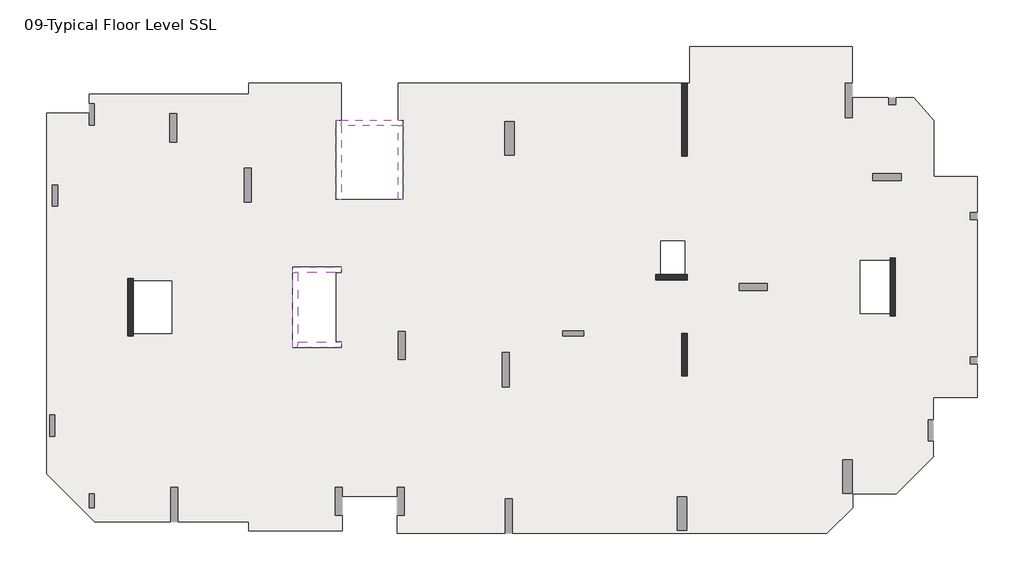
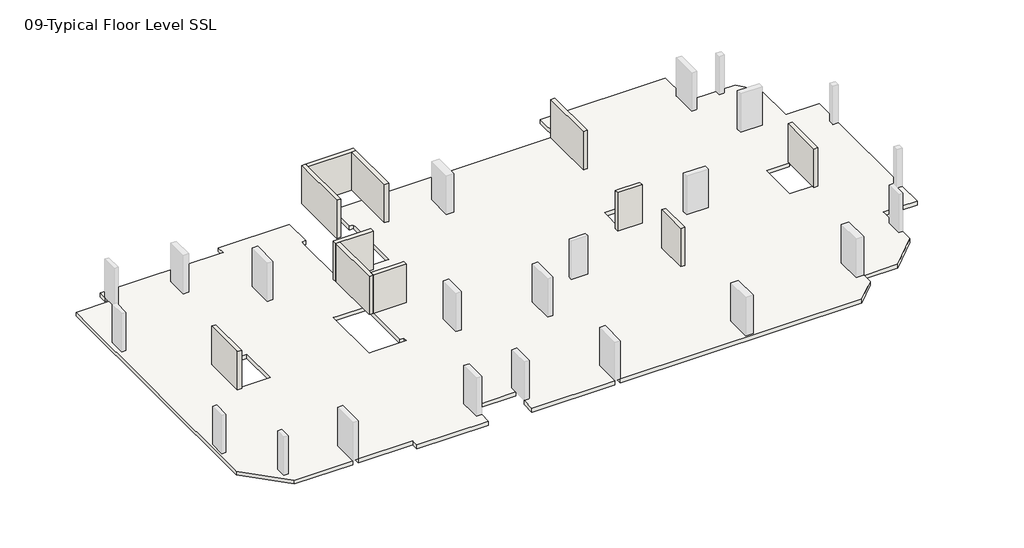
# One storey, part 1 of 2: 11 walls, 1 slab.
"""IFC4 building model written with IfcOpenShell, lengths in millimetres."""

from ifc_helpers import new_model, si_unit, origin, place, context, project, spatial, faceted_brep, element, save

model = new_model("IFC4")

# Units and contexts
model_context = context("Model", 3, world=origin())
ifc_project = project(units=[si_unit("LENGTHUNIT", "METRE", prefix="MILLI")], contexts=[model_context])

# Site, building, storey
site = spatial("IfcSite", under=ifc_project)
building = spatial("IfcBuilding", under=site)
storey = spatial("IfcBuildingStorey", under=building, Name="09-Typical Floor Level SSL", Elevation=21000.0)

# Slab
placement = place(None, origin())
element("IfcSlab", 1, ObjectType="Generic 300mm", at=placement, inside=storey, context=model_context, shape_type="Brep", body=[
    faceted_brep([(36192.0021644, 24072.000519, 20700.0), (36192.0021644, 26172.000519, 20700.0), (45446.0007483, 26172.000519, 20700.0), (45446.0007483, 24087.0, 20700.0), (45046.0007483, 24087.0, 20700.0), (45046.0007483, 22137.0, 20700.0), (45446.0007483, 22137.0, 20700.0), (45446.0007483, 23252.0000315, 20700.0), (47498.6337868, 23252.0000315, 20700.0), (47498.6337868, 22852.0, 20700.0), (47898.6337868, 22852.0, 20700.0), (47898.6337868, 23252.0000315, 20700.0), (48936.764334, 23252.0000315, 20700.0), (50076.0016214, 21956.8283806, 20700.0), (50076.0016214, 18780.0084406, 20700.0), (52549.9999998, 18780.0084406, 20700.0), (52549.9999998, 16712.0, 20700.0), (52149.9999998, 16712.0, 20700.0), (52149.9999998, 16312.0, 20700.0), (52549.9999998, 16312.0, 20700.0), (52549.9999998, 8504.0039609, 20700.0), (52149.9999998, 8504.0039609, 20700.0), (52149.9999998, 8104.0039609, 20700.0), (52549.9999998, 8104.0039609, 20700.0), (52549.9999998, 6204.0084406, 20700.0), (50046.0009271, 6204.0084406, 20700.0), (50046.0009271, 4931.9999929, 20700.0), (49746.0009271, 4931.9999929, 20700.0), (49746.0009271, 3731.9999929, 20700.0), (50046.0009271, 3731.9999929, 20700.0), (50046.0009271, 2810.5958657, 20700.0), (47943.4055804, 708.000519, 20700.0), (45456.0017287, 708.000519, 20700.0), (45456.0017287, -61.7051085, 20700.0), (43990.7023722, -1527.004465, 20700.0), (26113.9999998, -1527.004465, 20700.0), (26113.9999998, 422.995535, 20700.0), (25713.9999998, 422.995535, 20700.0), (25713.9999998, -1527.004465, 20700.0), (19569.9997488, -1527.004465, 20700.0), (19569.9997488, -512.0044652, 20700.0), (19969.9997488, -512.0044652, 20700.0), (19969.9997488, 1087.9955348, 20700.0), (19569.9997488, 1087.9955348, 20700.0), (19569.9997488, 564.000519, 20700.0), (16429.9999981, 564.000519, 20700.0), (16429.9999981, 1088.0, 20700.0), (16029.9999981, 1088.0, 20700.0), (16029.9999981, -512.0, 20700.0), (16429.9999981, -512.0, 20700.0), (16429.9999981, -1391.999481, 20700.0), (11136.0000923, -1391.999481, 20700.0), (11136.0000923, -866.9999847, 20700.0), (7082.0000416, -866.9999847, 20700.0), (7082.0000416, 1083.0000153, 20700.0), (6682.0000416, 1083.0000153, 20700.0), (6682.0000416, -866.9999847, 20700.0), (2364.4419097, -866.9999847, 20700.0), (-372.0, 1869.441925, 20700.0), (-372.0, 22380.0004589, 20700.0), (2052.0, 22380.0004589, 20700.0), (2052.0, 21708.0000656, 20700.0), (2352.0, 21708.0000656, 20700.0), (2352.0, 22908.0000656, 20700.0), (2052.0, 22908.0000656, 20700.0), (2052.0, 23472.000519, 20700.0), (11136.0000923, 23472.000519, 20700.0), (11136.0000923, 24072.000519, 20700.0), (16380.0000168, 24072.000519, 20700.0), (16380.0000168, 21972.0, 20700.0), (16079.9999997, 21972.0, 20700.0), (16079.9999997, 21672.0, 20700.0), (16079.9999997, 17468.0, 20700.0), (16379.9999997, 17468.0, 20700.0), (19619.9999997, 17468.0, 20700.0), (19919.9999997, 17468.0, 20700.0), (19919.9999997, 21672.0, 20700.0), (19919.9999997, 21972.0, 20700.0), (19619.9997365, 21972.0, 20700.0), (19619.9997365, 24072.000519, 20700.0), (35747.9999998, 24072.000519, 20700.0), (35747.9999998, 19932.0, 20700.0), (36047.9999998, 19932.0, 20700.0), (36047.9999998, 24072.000519, 20700.0), (16079.9999907, 9359.999998, 20700.0), (16079.9999907, 13320.0000002, 20700.0), (16380.0000168, 13320.0000002, 20700.0), (16380.0000168, 13620.0000002, 20700.0), (13919.9999907, 13620.0000002, 20700.0), (13619.9999907, 13620.0000002, 20700.0), (13619.9999907, 13320.0000002, 20700.0), (13619.9999907, 9359.999998, 20700.0), (13619.9999907, 9059.999998, 20700.0), (13919.9999907, 9059.999998, 20700.0), (16380.0000168, 9059.999998, 20700.0), (16380.0000168, 9359.999998, 20700.0), (4548.0000034, 9840.0000003, 20700.0), (6743.9999995, 9840.0000003, 20700.0), (6743.9999995, 12840.0000003, 20700.0), (4548.0000034, 12840.0000003, 20700.0), (4548.0000025, 12984.0000001, 20700.0), (4248.0000025, 12984.0000001, 20700.0), (4248.0000025, 9696.0, 20700.0), (4548.0000025, 9696.0, 20700.0), (47580.0014798, 13992.0079177, 20700.0), (45900.001729, 13992.0079177, 20700.0), (45900.001729, 10992.0079181, 20700.0), (47580.0014798, 10992.0079181, 20700.0), (47580.0014811, 10848.0079202, 20700.0), (47880.0014811, 10848.0079202, 20700.0), (47880.0014811, 14136.0000002, 20700.0), (47580.0014811, 14136.0000002, 20700.0), (35904.002157, 15108.0000083, 20700.0), (34548.0015145, 15108.0000083, 20700.0), (34548.0015145, 13199.9999992, 20700.0), (34248.0015201, 13199.9999992, 20700.0), (34248.0015201, 12899.9999992, 20700.0), (36048.0015201, 12899.9999992, 20700.0), (36048.0015201, 13199.9999992, 20700.0), (35904.002157, 13199.9999992, 20700.0), (257.9999999, 17088.0, 20700.0), (257.9999999, 18288.0, 20700.0), (-42.0000001, 18288.0, 20700.0), (-42.0000001, 17088.0, 20700.0), (108.001803, 4001.9999858, 20700.0), (108.001803, 5201.9999858, 20700.0), (-191.998197, 5201.9999858, 20700.0), (-191.998197, 4001.9999858, 20700.0), (30175.9999998, 9996.0000019, 20700.0), (28975.9999998, 9996.0000019, 20700.0), (28975.9999998, 9696.0000019, 20700.0), (30175.9999998, 9696.0000019, 20700.0), (7021.9999999, 20740.0000078, 20700.0), (7021.9999999, 22340.0000078, 20700.0), (6621.9999999, 22340.0000078, 20700.0), (6621.9999999, 20740.0000078, 20700.0), (48205.9993605, 18950.0, 20700.0), (46605.9993605, 18950.0, 20700.0), (46605.9993605, 18550.0, 20700.0), (48205.9993605, 18550.0, 20700.0), (20030.000009, 8355.9999979, 20700.0), (20030.000009, 9955.9999979, 20700.0), (19630.000009, 9955.9999979, 20700.0), (19630.000009, 8355.9999979, 20700.0), (11270.0000427, 17312.9999996, 20700.0), (11270.0000427, 19262.9999996, 20700.0), (10870.0000427, 19262.9999996, 20700.0), (10870.0000427, 17312.9999996, 20700.0), (40598.0014887, 12692.0079212, 20700.0), (38998.0014887, 12692.0079212, 20700.0), (38998.0014887, 12292.0079212, 20700.0), (40598.0014887, 12292.0079212, 20700.0), (2352.0, -72.0, 20700.0), (2352.0, 728.0, 20700.0), (2052.0, 728.0, 20700.0), (2052.0, -72.0, 20700.0), (25934.0000455, 6801.0001824, 20700.0), (25934.0000455, 8751.0001824, 20700.0), (25534.0000455, 8751.0001824, 20700.0), (25534.0000455, 6801.0001824, 20700.0), (36035.9999998, -1351.9992017, 20700.0), (36035.9999998, 548.0007983, 20700.0), (35485.9999998, 548.0007983, 20700.0), (35485.9999998, -1351.9992017, 20700.0), (45443.9999998, 748.0, 20700.0), (45443.9999998, 2648.0, 20700.0), (44893.9999998, 2648.0, 20700.0), (44893.9999998, 748.0, 20700.0), (26218.9999998, 20000.0, 20700.0), (26218.9999998, 21900.0, 20700.0), (25668.9999998, 21900.0, 20700.0), (25668.9999998, 20000.0, 20700.0), (35748.0054035, 9840.0000002, 20700.0), (35748.0054035, 7428.0000762, 20700.0), (36048.0054035, 7428.0000762, 20700.0), (36048.0054035, 9840.0000002, 20700.0), (36192.0021644, 26172.000519, 21000.0), (36192.0021644, 24072.000519, 21000.0), (36047.9999998, 24072.000519, 21000.0), (36047.9999998, 19932.0, 21000.0), (35747.9999998, 19932.0, 21000.0), (35747.9999998, 24072.000519, 21000.0), (19619.9997365, 24072.000519, 21000.0), (19619.9997365, 21972.0, 21000.0), (19919.9999997, 21972.0, 21000.0), (19919.9999997, 21672.0, 21000.0), (19919.9999997, 17468.0, 21000.0), (19619.9999997, 17468.0, 21000.0), (16379.9999997, 17468.0, 21000.0), (16079.9999997, 17468.0, 21000.0), (16079.9999997, 21672.0, 21000.0), (16079.9999997, 21972.0, 21000.0), (16380.0000168, 21972.0, 21000.0), (16380.0000168, 24072.000519, 21000.0), (11136.0000923, 24072.000519, 21000.0), (11136.0000923, 23472.000519, 21000.0), (2052.0, 23472.000519, 21000.0), (2052.0, 22908.0000656, 21000.0), (2352.0, 22908.0000656, 21000.0), (2352.0, 21708.0000656, 21000.0), (2052.0, 21708.0000656, 21000.0), (2052.0, 22380.0004589, 21000.0), (-372.0, 22380.0004589, 21000.0), (-372.0, 1869.441925, 21000.0), (2364.4419097, -866.9999847, 21000.0), (6682.0000416, -866.9999847, 21000.0), (6682.0000416, 1083.0000153, 21000.0), (7082.0000416, 1083.0000153, 21000.0), (7082.0000416, -866.9999847, 21000.0), (11136.0000923, -866.9999847, 21000.0), (11136.0000923, -1391.999481, 21000.0), (16429.9999981, -1391.999481, 21000.0), (16429.9999981, -512.0, 21000.0), (16029.9999981, -512.0, 21000.0), (16029.9999981, 1088.0, 21000.0), (16429.9999981, 1088.0, 21000.0), (16429.9999981, 564.000519, 21000.0), (19569.9997488, 564.000519, 21000.0), (19569.9997488, 1087.9955348, 21000.0), (19969.9997488, 1087.9955348, 21000.0), (19969.9997488, -512.0044652, 21000.0), (19569.9997488, -512.0044652, 21000.0), (19569.9997488, -1527.004465, 21000.0), (25713.9999998, -1527.004465, 21000.0), (25713.9999998, 422.995535, 21000.0), (26113.9999998, 422.995535, 21000.0), (26113.9999998, -1527.004465, 21000.0), (43990.7023722, -1527.004465, 21000.0), (45456.0017287, -61.7051085, 21000.0), (45456.0017287, 708.000519, 21000.0), (47943.4055804, 708.000519, 21000.0), (50046.0009271, 2810.5958657, 21000.0), (50046.0009271, 3731.9999929, 21000.0), (49746.0009271, 3731.9999929, 21000.0), (49746.0009271, 4931.9999929, 21000.0), (50046.0009271, 4931.9999929, 21000.0), (50046.0009271, 6204.0084406, 21000.0), (52549.9999998, 6204.0084406, 21000.0), (52549.9999998, 8104.0039609, 21000.0), (52149.9999998, 8104.0039609, 21000.0), (52149.9999998, 8504.0039609, 21000.0), (52549.9999998, 8504.0039609, 21000.0), (52549.9999998, 16312.0, 21000.0), (52149.9999998, 16312.0, 21000.0), (52149.9999998, 16712.0, 21000.0), (52549.9999998, 16712.0, 21000.0), (52549.9999998, 18780.0084406, 21000.0), (50076.0016214, 18780.0084406, 21000.0), (50076.0016214, 21956.8283806, 21000.0), (48936.764334, 23252.0000315, 21000.0), (47898.6337868, 23252.0000315, 21000.0), (47898.6337868, 22852.0, 21000.0), (47498.6337868, 22852.0, 21000.0), (47498.6337868, 23252.0000315, 21000.0), (45446.0006898, 23252.0000315, 21000.0), (45446.0007483, 22137.0, 21000.0), (45046.0007483, 22137.0, 21000.0), (45046.0007483, 24087.0, 21000.0), (45446.0007483, 24087.0, 21000.0), (45446.0007483, 26172.000519, 21000.0), (16079.9999907, 13320.0000002, 21000.0), (16079.9999907, 9359.999998, 21000.0), (16380.0000168, 9359.999998, 21000.0), (16380.0000168, 9059.999998, 21000.0), (13919.9999907, 9059.999998, 21000.0), (13619.9999907, 9059.999998, 21000.0), (13619.9999907, 9359.999998, 21000.0), (13619.9999907, 13320.0000002, 21000.0), (13619.9999907, 13620.0000002, 21000.0), (13919.9999907, 13620.0000002, 21000.0), (16380.0000168, 13620.0000002, 21000.0), (16380.0000168, 13320.0000002, 21000.0), (6743.9999995, 9840.0000003, 21000.0), (4548.0000034, 9840.0000003, 21000.0), (4548.0000025, 9696.0, 21000.0), (4248.0000025, 9696.0, 21000.0), (4248.0000025, 12984.0000001, 21000.0), (4548.0000025, 12984.0000001, 21000.0), (4548.0000025, 12840.0000003, 21000.0), (6743.9999995, 12840.0000003, 21000.0), (45900.001729, 13992.0079177, 21000.0), (47580.0014798, 13992.0079177, 21000.0), (47580.0014811, 14136.0000002, 21000.0), (47880.0014811, 14136.0000002, 21000.0), (47880.0014811, 10848.0079202, 21000.0), (47580.0014811, 10848.0079202, 21000.0), (47580.0014811, 10992.0079181, 21000.0), (45900.001729, 10992.0079181, 21000.0), (34548.0015145, 15108.0000083, 21000.0), (35904.002157, 15108.0000083, 21000.0), (35904.002157, 13199.9999992, 21000.0), (36048.0015201, 13199.9999992, 21000.0), (36048.0015201, 12899.9999992, 21000.0), (34248.0015201, 12899.9999992, 21000.0), (34248.0015201, 13199.9999992, 21000.0), (34548.0015145, 13199.9999992, 21000.0), (257.9999999, 18288.0, 21000.0), (257.9999999, 17088.0, 21000.0), (-42.0000001, 17088.0, 21000.0), (-42.0000001, 18288.0, 21000.0), (108.001803, 5201.9999858, 21000.0), (108.001803, 4001.9999858, 21000.0), (-191.998197, 4001.9999858, 21000.0), (-191.998197, 5201.9999858, 21000.0), (28975.9999998, 9996.0000019, 21000.0), (30175.9999998, 9996.0000019, 21000.0), (30175.9999998, 9696.0000019, 21000.0), (28975.9999998, 9696.0000019, 21000.0), (7021.9999999, 22340.0000078, 21000.0), (7021.9999999, 20740.0000078, 21000.0), (6621.9999999, 20740.0000078, 21000.0), (6621.9999999, 22340.0000078, 21000.0), (46605.9993605, 18950.0, 21000.0), (48205.9993605, 18950.0, 21000.0), (48205.9993605, 18550.0, 21000.0), (46605.9993605, 18550.0, 21000.0), (20030.000009, 9955.9999979, 21000.0), (20030.000009, 8355.9999979, 21000.0), (19630.000009, 8355.9999979, 21000.0), (19630.000009, 9955.9999979, 21000.0), (11270.0000427, 19262.9999996, 21000.0), (11270.0000427, 17312.9999996, 21000.0), (10870.0000427, 17312.9999996, 21000.0), (10870.0000427, 19262.9999996, 21000.0), (38998.0014887, 12692.0079212, 21000.0), (40598.0014887, 12692.0079212, 21000.0), (40598.0014887, 12292.0079212, 21000.0), (38998.0014887, 12292.0079212, 21000.0), (2352.0, 728.0, 21000.0), (2352.0, -72.0, 21000.0), (2052.0, -72.0, 21000.0), (2052.0, 728.0, 21000.0), (25934.0000455, 8751.0001824, 21000.0), (25934.0000455, 6801.0001824, 21000.0), (25534.0000455, 6801.0001824, 21000.0), (25534.0000455, 8751.0001824, 21000.0), (36035.9999998, 548.0007983, 21000.0), (36035.9999998, -1351.9992017, 21000.0), (35485.9999998, -1351.9992017, 21000.0), (35485.9999998, 548.0007983, 21000.0), (45443.9999998, 2648.0, 21000.0), (45443.9999998, 748.0, 21000.0), (44893.9999998, 748.0, 21000.0), (44893.9999998, 2648.0, 21000.0), (26218.9999998, 21900.0, 21000.0), (26218.9999998, 20000.0, 21000.0), (25668.9999998, 20000.0, 21000.0), (25668.9999998, 21900.0, 21000.0), (35748.0054035, 7428.0000762, 21000.0), (35748.0054035, 9840.0000002, 21000.0), (36048.0054035, 9840.0000002, 21000.0), (36048.0054035, 7428.0000762, 21000.0)], [[[0, 1, 2, 3, 4, 5, 6, 7, 8, 9, 10, 11, 12, 13, 14, 15, 16, 17, 18, 19, 20, 21, 22, 23, 24, 25, 26, 27, 28, 29, 30, 31, 32, 33, 34, 35, 36, 37, 38, 39, 40, 41, 42, 43, 44, 45, 46, 47, 48, 49, 50, 51, 52, 53, 54, 55, 56, 57, 58, 59, 60, 61, 62, 63, 64, 65, 66, 67, 68, 69, 70, 71, 72, 73, 74, 75, 76, 77, 78, 79, 80, 81, 82, 83], [84, 85, 86, 87, 88, 89, 90, 91, 92, 93, 94, 95], [96, 97, 98, 99, 100, 101, 102, 103], [104, 105, 106, 107, 108, 109, 110, 111], [112, 113, 114, 115, 116, 117, 118, 119], [120, 121, 122, 123], [124, 125, 126, 127], [128, 129, 130, 131], [132, 133, 134, 135], [136, 137, 138, 139], [140, 141, 142, 143], [144, 145, 146, 147], [148, 149, 150, 151], [152, 153, 154, 155], [156, 157, 158, 159], [160, 161, 162, 163], [164, 165, 166, 167], [168, 169, 170, 171], [172, 173, 174, 175]], [[176, 177, 178, 179, 180, 181, 182, 183, 184, 185, 186, 187, 188, 189, 190, 191, 192, 193, 194, 195, 196, 197, 198, 199, 200, 201, 202, 203, 204, 205, 206, 207, 208, 209, 210, 211, 212, 213, 214, 215, 216, 217, 218, 219, 220, 221, 222, 223, 224, 225, 226, 227, 228, 229, 230, 231, 232, 233, 234, 235, 236, 237, 238, 239, 240, 241, 242, 243, 244, 245, 246, 247, 248, 249, 250, 251, 252, 253, 254, 255, 256, 257, 258, 259], [260, 261, 262, 263, 264, 265, 266, 267, 268, 269, 270, 271], [272, 273, 274, 275, 276, 277, 278, 279], [280, 281, 282, 283, 284, 285, 286, 287], [288, 289, 290, 291, 292, 293, 294, 295], [296, 297, 298, 299], [300, 301, 302, 303], [304, 305, 306, 307], [308, 309, 310, 311], [312, 313, 314, 315], [316, 317, 318, 319], [320, 321, 322, 323], [324, 325, 326, 327], [328, 329, 330, 331], [332, 333, 334, 335], [336, 337, 338, 339], [340, 341, 342, 343], [344, 345, 346, 347], [348, 349, 350, 351]], [[68, 193, 192, 69]], [[182, 79, 78, 183]], [[79, 182, 181, 80]], [[177, 0, 83, 178]], [[1, 0, 177, 176]], [[2, 1, 176, 259]], [[3, 2, 259, 258]], [[249, 12, 11, 250]], [[7, 254, 253, 8]], [[13, 12, 249, 248]], [[14, 13, 248, 247]], [[15, 14, 247, 246]], [[15, 246, 245, 16]], [[237, 24, 23, 238]], [[19, 242, 241, 20]], [[25, 24, 237, 236]], [[25, 236, 235, 26]], [[231, 30, 29, 232]], [[32, 31, 230, 229]], [[33, 32, 229, 228]], [[34, 33, 228, 227]], [[34, 227, 226, 35]], [[222, 39, 38, 223]], [[39, 222, 221, 40]], [[45, 44, 217, 216]], [[211, 50, 49, 212]], [[51, 50, 211, 210]], [[52, 51, 210, 209]], [[52, 209, 208, 53]], [[204, 57, 56, 205]], [[58, 57, 204, 203]], [[59, 58, 203, 202]], [[60, 59, 202, 201]], [[196, 65, 64, 197]], [[66, 65, 196, 195]], [[67, 66, 195, 194]], [[68, 67, 194, 193]], [[31, 30, 231, 230]], [[85, 84, 261, 260]], [[72, 189, 188, 187, 186, 75, 74, 73]], [[272, 97, 96, 273]], [[97, 272, 279, 98]], [[98, 279, 278, 99]], [[280, 105, 104, 281]], [[105, 280, 287, 106]], [[106, 287, 286, 107]], [[112, 289, 288, 113]], [[113, 288, 295, 114]], [[289, 112, 119, 290]], [[62, 199, 198, 63]], [[199, 62, 61, 200]], [[200, 61, 60, 201]], [[63, 198, 197, 64]], [[120, 297, 296, 121]], [[297, 120, 123, 298]], [[298, 123, 122, 299]], [[299, 122, 121, 296]], [[124, 301, 300, 125]], [[301, 124, 127, 302]], [[302, 127, 126, 303]], [[303, 126, 125, 300]], [[28, 233, 232, 29]], [[233, 28, 27, 234]], [[234, 27, 26, 235]], [[128, 305, 304, 129]], [[305, 128, 131, 306]], [[306, 131, 130, 307]], [[307, 130, 129, 304]], [[132, 309, 308, 133]], [[309, 132, 135, 310]], [[310, 135, 134, 311]], [[311, 134, 133, 308]], [[41, 220, 219, 42]], [[220, 41, 40, 221]], [[43, 218, 217, 44]], [[218, 43, 42, 219]], [[136, 313, 312, 137]], [[313, 136, 139, 314]], [[314, 139, 138, 315]], [[315, 138, 137, 312]], [[140, 317, 316, 141]], [[317, 140, 143, 318]], [[318, 143, 142, 319]], [[319, 142, 141, 316]], [[215, 46, 45, 216]], [[48, 213, 212, 49]], [[213, 48, 47, 214]], [[214, 47, 46, 215]], [[144, 321, 320, 145]], [[321, 144, 147, 322]], [[322, 147, 146, 323]], [[323, 146, 145, 320]], [[207, 54, 53, 208]], [[55, 206, 205, 56]], [[206, 55, 54, 207]], [[225, 36, 35, 226]], [[37, 224, 223, 38]], [[224, 37, 36, 225]], [[6, 255, 254, 7]], [[255, 6, 5, 256]], [[256, 5, 4, 257]], [[257, 4, 3, 258]], [[148, 325, 324, 149]], [[325, 148, 151, 326]], [[326, 151, 150, 327]], [[327, 150, 149, 324]], [[152, 329, 328, 153]], [[329, 152, 155, 330]], [[330, 155, 154, 331]], [[331, 154, 153, 328]], [[156, 333, 332, 157]], [[333, 156, 159, 334]], [[334, 159, 158, 335]], [[335, 158, 157, 332]], [[160, 337, 336, 161]], [[337, 160, 163, 338]], [[338, 163, 162, 339]], [[339, 162, 161, 336]], [[164, 341, 340, 165]], [[341, 164, 167, 342]], [[342, 167, 166, 343]], [[343, 166, 165, 340]], [[168, 345, 344, 169]], [[345, 168, 171, 346]], [[346, 171, 170, 347]], [[347, 170, 169, 344]], [[70, 191, 190, 189, 72, 71]], [[191, 70, 69, 192]], [[77, 184, 183, 78]], [[184, 77, 76, 75, 186, 185]], [[271, 86, 85, 260]], [[87, 270, 269, 268, 89, 88]], [[86, 271, 270, 87]], [[89, 268, 267, 266, 265, 92, 91, 90]], [[92, 265, 264, 263, 94, 93]], [[95, 262, 261, 84]], [[262, 95, 94, 263]], [[277, 100, 99, 278]], [[103, 274, 273, 96]], [[101, 276, 275, 102]], [[100, 277, 276, 101]], [[274, 103, 102, 275]], [[116, 293, 292, 117]], [[118, 291, 290, 119]], [[294, 115, 114, 295]], [[117, 292, 291, 118]], [[293, 116, 115, 294]], [[172, 349, 348, 173]], [[174, 351, 350, 175]], [[173, 348, 351, 174]], [[349, 172, 175, 350]], [[285, 108, 107, 286]], [[111, 282, 281, 104]], [[109, 284, 283, 110]], [[108, 285, 284, 109]], [[282, 111, 110, 283]], [[82, 179, 178, 83]], [[180, 81, 80, 181]], [[179, 82, 81, 180]], [[18, 243, 242, 19]], [[243, 18, 17, 244]], [[244, 17, 16, 245]], [[10, 251, 250, 11]], [[251, 10, 9, 252]], [[252, 9, 8, 253]], [[22, 239, 238, 23]], [[239, 22, 21, 240]], [[240, 21, 20, 241]]]),
])

# Walls
element("IfcWall", 2, ObjectType="Shear Walls 300mm", at=placement, inside=storey, context=model_context, shape_type="Brep", body=[
    faceted_brep([(4548.0000025, 9696.0, 21000.0), (4548.0000025, 12984.0000001, 21000.0), (4548.0000025, 12984.0000001, 23700.0), (4548.0000025, 12984.0000001, 24000.0), (4548.0000025, 12840.0000003, 24000.0), (4548.0000025, 9840.0000003, 24000.0), (4548.0000025, 9696.0, 24000.0), (4548.0000025, 9696.0, 23700.0), (4248.0000025, 9696.0, 21000.0), (4248.0000025, 9696.0, 23700.0), (4248.0000025, 9696.0, 24000.0), (4248.0000025, 12984.0000001, 24000.0), (4248.0000025, 12984.0000001, 23700.0), (4248.0000025, 12984.0000001, 21000.0)], [[[0, 1, 2, 3, 4, 5, 6, 7]], [[8, 9, 10, 11, 12, 13]], [[1, 0, 8, 13]], [[3, 2, 1, 13, 12, 11]], [[6, 5, 4, 3, 11, 10]], [[0, 7, 6, 10, 9, 8]]]),
])
element("IfcWall", 3, ObjectType="Shear Walls 300mm", at=placement, inside=storey, context=model_context, shape_type="Brep", body=[
    faceted_brep([(34248.0015201, 12899.9999992, 21000.0), (36048.0015201, 12899.9999992, 21000.0), (36048.0015201, 12899.9999992, 23700.0), (36048.0015201, 12899.9999992, 24000.0), (34248.0015201, 12899.9999992, 24000.0), (34248.0015201, 12899.9999992, 23700.0), (34248.0015201, 13199.9999992, 21000.0), (34248.0015201, 13199.9999992, 23700.0), (34248.0015201, 13199.9999992, 24000.0), (34548.0015145, 13199.9999992, 24000.0), (35904.002157, 13199.9999992, 24000.0), (36048.0015201, 13199.9999992, 24000.0), (36048.0015201, 13199.9999992, 23700.0), (36048.0015201, 13199.9999992, 21000.0)], [[[0, 1, 2, 3, 4, 5]], [[6, 7, 8, 9, 10, 11, 12, 13]], [[1, 0, 6, 13]], [[3, 2, 1, 13, 12, 11]], [[4, 3, 11, 10, 9, 8]], [[0, 5, 4, 8, 7, 6]]]),
])
element("IfcWall", 4, ObjectType="Shear Walls 300mm", at=placement, inside=storey, context=model_context, shape_type="Brep", body=[
    faceted_brep([(35748.0054035, 9840.0000002, 21000.0), (35748.0054035, 7428.0000762, 21000.0), (35748.0054035, 7428.0000762, 23700.0), (35748.0054035, 7428.0000762, 24000.0), (35748.0054035, 9840.0000002, 24000.0), (35748.0054035, 9840.0000002, 23700.0), (36048.0054035, 9840.0000002, 21000.0), (36048.0054035, 9840.0000002, 23700.0), (36048.0054035, 9840.0000002, 24000.0), (36048.0054035, 7428.0000762, 24000.0), (36048.0054035, 7428.0000762, 23700.0), (36048.0054035, 7428.0000762, 21000.0)], [[[0, 1, 2, 3, 4, 5]], [[6, 7, 8, 9, 10, 11]], [[1, 0, 6, 11]], [[3, 2, 1, 11, 10, 9]], [[4, 3, 9, 8]], [[0, 5, 4, 8, 7, 6]]]),
])
element("IfcWall", 5, ObjectType="Shear Walls 300mm", at=placement, inside=storey, context=model_context, shape_type="Brep", body=[
    faceted_brep([(47580.0014811, 14136.0000002, 21000.0), (47580.0014811, 10848.0079202, 21000.0), (47580.0014811, 10848.0079202, 23700.0), (47580.0014811, 10848.0079202, 24000.0), (47580.0014811, 10992.0079181, 24000.0), (47580.0014811, 13992.0079177, 24000.0), (47580.0014811, 14136.0000002, 24000.0), (47580.0014811, 14136.0000002, 23700.0), (47880.0014811, 14136.0000002, 21000.0), (47880.0014811, 14136.0000002, 23700.0), (47880.0014811, 14136.0000002, 24000.0), (47880.0014811, 10848.0079202, 24000.0), (47880.0014811, 10848.0079202, 23700.0), (47880.0014811, 10848.0079202, 21000.0)], [[[0, 1, 2, 3, 4, 5, 6, 7]], [[8, 9, 10, 11, 12, 13]], [[1, 0, 8, 13]], [[3, 2, 1, 13, 12, 11]], [[6, 5, 4, 3, 11, 10]], [[0, 7, 6, 10, 9, 8]]]),
])
element("IfcWall", 6, ObjectType="Shear Walls 300mm", at=placement, inside=storey, context=model_context, shape_type="Brep", body=[
    faceted_brep([(36047.9999998, 19932.0, 21000.0), (36047.9999998, 24072.0078999, 21000.0), (36047.9999998, 24072.0078999, 24000.0), (36047.9999998, 19932.0, 24000.0), (36047.9999998, 19932.0, 23700.0), (35747.9999998, 19932.0, 21000.0), (35747.9999998, 19932.0, 23700.0), (35747.9999998, 19932.0, 24000.0), (35747.9999998, 24072.0078999, 24000.0), (35747.9999998, 24072.0078999, 21000.0)], [[[0, 1, 2, 3, 4]], [[5, 6, 7, 8, 9]], [[1, 0, 5, 9]], [[2, 1, 9, 8]], [[3, 2, 8, 7]], [[0, 4, 3, 7, 6, 5]]]),
])
element("IfcWall", 7, ObjectType="Shear Walls 300mm", at=placement, inside=storey, context=model_context, shape_type="Brep", body=[
    faceted_brep([(16379.9999997, 21972.0, 27000.0), (16379.9999997, 21672.0, 27000.0), (16379.9999997, 17468.0, 27000.0), (16379.9999997, 17468.0, 24000.0), (16379.9999997, 21672.0, 24000.0), (16379.9999997, 21972.0, 24000.0), (16079.9999997, 17468.0, 27000.0), (16079.9999997, 21972.0, 27000.0), (16079.9999997, 21972.0, 26700.0), (16079.9999997, 21972.0, 24000.0), (16079.9999997, 17468.0, 24000.0), (16079.9999997, 17468.0, 26700.0)], [[[0, 1, 2, 3, 4, 5]], [[6, 7, 8, 9, 10, 11]], [[2, 1, 0, 7, 6]], [[2, 6, 11, 10, 3]], [[3, 10, 9, 5, 4]], [[0, 5, 9, 8, 7]]]),
])
element("IfcWall", 8, ObjectType="Shear Walls 300mm", at=placement, inside=storey, context=model_context, shape_type="Brep", body=[
    faceted_brep([(16379.9999997, 21972.0, 27000.0), (19619.9997365, 21972.0, 27000.0), (19919.9999997, 21972.0, 27000.0), (19919.9999997, 21972.0, 26700.0), (19919.9999997, 21972.0, 24000.0), (16379.9999997, 21972.0, 24000.0), (19919.9999997, 21672.0, 27000.0), (19619.9999997, 21672.0, 27000.0), (16379.9999997, 21672.0, 27000.0), (16379.9999997, 21672.0, 24000.0), (19619.9999997, 21672.0, 24000.0), (19919.9999997, 21672.0, 24000.0)], [[[0, 1, 2, 3, 4, 5]], [[6, 7, 8, 9, 10, 11]], [[2, 1, 0, 8, 7, 6]], [[8, 0, 5, 9]], [[9, 5, 4, 11, 10]], [[4, 3, 2, 6, 11]]]),
])
element("IfcWall", 9, ObjectType="Shear Walls 300mm", at=placement, inside=storey, context=model_context, shape_type="Brep", body=[
    faceted_brep([(19919.9999997, 21672.0, 27000.0), (19919.9999997, 17468.0, 27000.0), (19919.9999997, 17468.0, 26700.0), (19919.9999997, 17468.0, 24000.0), (19919.9999997, 21672.0, 24000.0), (19619.9999997, 17468.0, 27000.0), (19619.9999997, 21672.0, 27000.0), (19619.9999997, 21672.0, 24000.0), (19619.9999997, 17468.0, 24000.0)], [[[0, 1, 2, 3, 4]], [[5, 6, 7, 8]], [[1, 0, 6, 5]], [[1, 5, 8, 3, 2]], [[6, 0, 4, 7]], [[4, 3, 8, 7]]]),
])
element("IfcWall", 10, ObjectType="Shear Walls 300mm", at=placement, inside=storey, context=model_context, shape_type="Brep", body=[
    faceted_brep([(16380.0000168, 13320.0000002, 27000.0), (16079.9999907, 13320.0000002, 27000.0), (13919.9999907, 13320.0000002, 27000.0), (13619.9999907, 13320.0000002, 27000.0), (13619.9999907, 13320.0000002, 24000.0), (13919.9999907, 13320.0000002, 24000.0), (16380.0000168, 13320.0000002, 24000.0), (16380.0000168, 13320.0000002, 26700.0), (13619.9999907, 13620.0000002, 27000.0), (16380.0000168, 13620.0000002, 27000.0), (16380.0000168, 13620.0000002, 26700.0), (16380.0000168, 13620.0000002, 24000.0), (13619.9999907, 13620.0000002, 24000.0), (13619.9999907, 13620.0000002, 26700.0)], [[[0, 1, 2, 3, 4, 5, 6, 7]], [[8, 9, 10, 11, 12, 13]], [[9, 0, 7, 6, 11, 10]], [[3, 2, 1, 0, 9, 8]], [[11, 6, 5, 4, 12]], [[4, 3, 8, 13, 12]]]),
])
element("IfcWall", 11, ObjectType="Shear Walls 300mm", at=placement, inside=storey, context=model_context, shape_type="Brep", body=[
    faceted_brep([(13919.9999907, 13320.0000002, 27000.0), (13919.9999907, 9359.999998, 27000.0), (13919.9999907, 9059.999998, 27000.0), (13919.9999907, 9059.999998, 24000.0), (13919.9999907, 9359.999998, 24000.0), (13919.9999907, 13320.0000002, 24000.0), (13619.9999907, 9059.999998, 27000.0), (13619.9999907, 13320.0000002, 27000.0), (13619.9999907, 13320.0000002, 24000.0), (13619.9999907, 9059.999998, 24000.0), (13619.9999907, 9059.999998, 26700.0)], [[[0, 1, 2, 3, 4, 5]], [[6, 7, 8, 9, 10]], [[2, 1, 0, 7, 6]], [[7, 0, 5, 8]], [[8, 5, 4, 3, 9]], [[3, 2, 6, 10, 9]]]),
])
element("IfcWall", 12, ObjectType="Shear Walls 300mm", at=placement, inside=storey, context=model_context, shape_type="Brep", body=[
    faceted_brep([(13919.9999907, 9359.999998, 27000.0), (16079.9999907, 9359.999998, 27000.0), (16380.0000168, 9359.999998, 27000.0), (16380.0000168, 9359.999998, 26700.0), (16380.0000168, 9359.999998, 24000.0), (13919.9999907, 9359.999998, 24000.0), (16380.0000168, 9059.999998, 27000.0), (13919.9999907, 9059.999998, 27000.0), (13919.9999907, 9059.999998, 24000.0), (16380.0000168, 9059.999998, 24000.0), (16380.0000168, 9059.999998, 26700.0)], [[[0, 1, 2, 3, 4, 5]], [[6, 7, 8, 9, 10]], [[2, 1, 0, 7, 6]], [[2, 6, 10, 9, 4, 3]], [[7, 0, 5, 8]], [[5, 4, 9, 8]]]),
])

save(model, "model.ifc")

# Revit data of these elements
# Type "Generic 300mm"
#   Function = 0
#   Layers, outside or top first: 300 mm "Concrete-RC" (function 1)
# Type "Shear Walls 300mm"
#   Layers, outside or top first: 300 mm "Concrete-RC" (function 1)
# Element 1 (IfcSlab, "Generic 300mm")
#   Height Offset From Level = 0 mm
#   built-in parameter 1001954 = 1
#   Phase Created = New Construction
#   Materials on its faces: "Concrete-RC"
# Elements 2, 3, 4, 5, 6 (IfcWall, "Shear Walls 300mm")
#   Top Offset = 0 mm
#   Base Offset = 0 mm
#   wall height = 3000 mm
#   Phase Created = New Construction
#   Base Constraint = 09-Typical Floor Level SSL
#   Top Constraint = 10-Typical Floor Level SSL
#   Materials on its faces: "Concrete-RC"
# Elements 7, 8, 9, 10, 11, 12 (IfcWall, "Shear Walls 300mm")
#   Top Offset = 0 mm
#   Base Offset = 0 mm
#   wall height = 6000 mm
#   Phase Created = New Construction
#   Base Constraint = 09-Typical Floor Level SSL
#   Top Constraint = 11-Typical Floor Level SSL
#   Materials on its faces: "Concrete-RC"
# Materials
#   "Concrete-RC": class "Concrete", colour RGB 128 128 128, transparency 0, Description = "High strength concrete", Cost = 0
